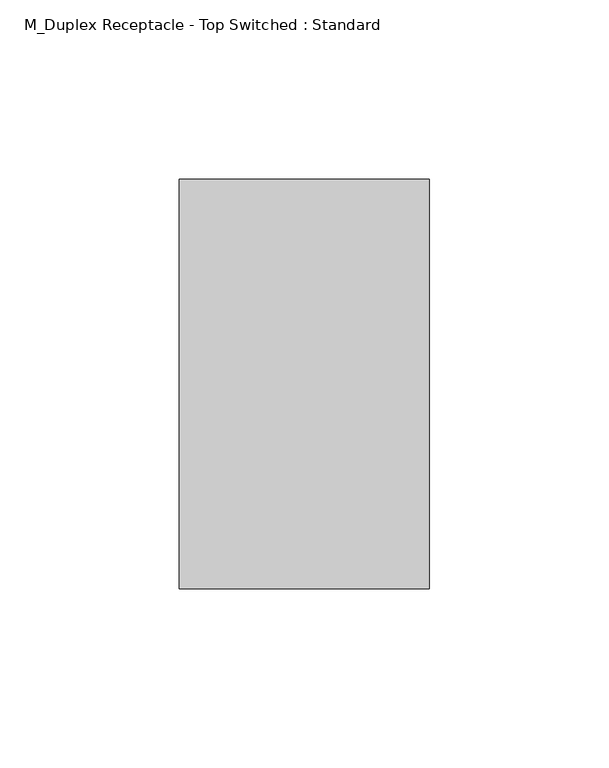
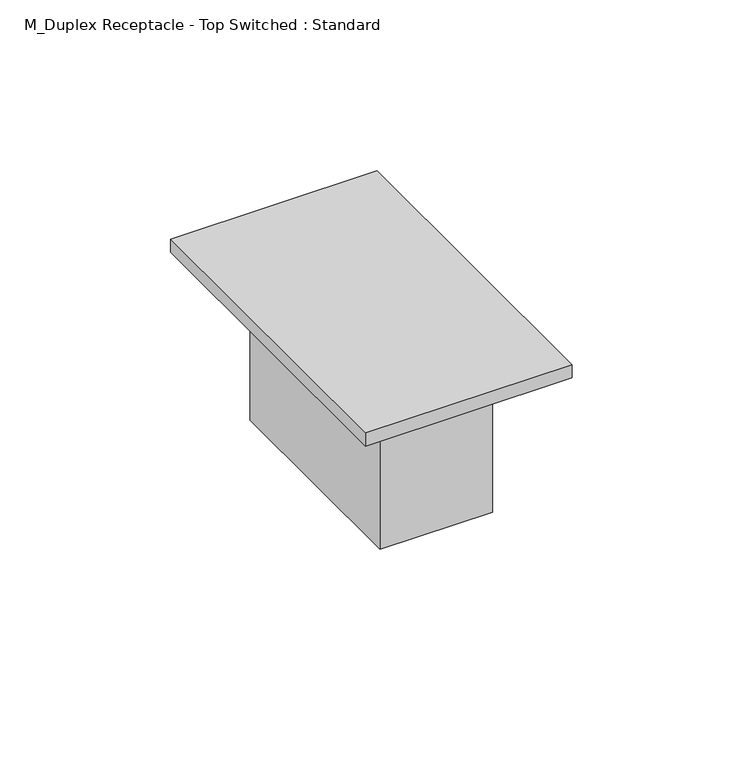
"""IFC4 building model written with IfcOpenShell, lengths in millimetres: proxy geometry, M_Duplex Receptacle - Top Switched : Standard."""

import ifcopenshell
import ifcopenshell.guid

model = None  # the IFC model being written
_history = None  # IfcOwnerHistory: only IFC2X3 demands one
_inside = {}  # id of a spatial element -> (the spatial element, [elements in it])
_under = {}  # id of a project, library or spatial element -> (it, [spatial elements below it])
_declared = {}  # id of a project -> (the project, [libraries it declares])
_typed = {}  # id of a type object -> (the type object, [elements of that type])
_made_of = {}  # id of a material, layer set ... -> (it, [elements and type objects made of it])


def new_model(schema):
    """Start an empty IFC model of exactly this schema.

    Asked for "IFC4X3", IfcOpenShell would pick the latest addendum, in which some entities
    have other attributes; the version numbers below select the first issue.
    IFC2X3 requires an IfcOwnerHistory on every rooted entity: one is made here for all.
    """
    global model, _history
    if schema == "IFC4X3":
        model = ifcopenshell.file(schema_version=(4, 3, 0, 0))
    else:
        model = ifcopenshell.file(schema=schema)
    _inside.clear()
    _under.clear()
    _declared.clear()
    _typed.clear()
    _made_of.clear()
    _history = None
    if model.schema == "IFC2X3":
        org = make("IfcOrganization", Name="unknown")
        user = make(
            "IfcPersonAndOrganization",
            ThePerson=make("IfcPerson", FamilyName="unknown"),
            TheOrganization=org,
        )
        app = make(
            "IfcApplication",
            ApplicationDeveloper=org,
            Version="unknown",
            ApplicationFullName="unknown",
            ApplicationIdentifier="unknown",
        )
        _history = make(
            "IfcOwnerHistory",
            OwningUser=user,
            OwningApplication=app,
            ChangeAction="ADDED",
            CreationDate=0,
        )
    return model


def make(cls, **values):
    """One entity of the class cls with the attributes given. An attribute that is None is left unset."""
    return model.create_entity(
        cls, **{name: value for name, value in values.items() if value is not None}
    )


def rooted(cls, **values):
    """An entity with a GlobalId (a new one), such as an element, a storey or a relation."""
    return make(cls, GlobalId=ifcopenshell.guid.new(), OwnerHistory=_history, **values)


def si_unit(unit_type, name, prefix=None):
    """IfcSIUnit, for example si_unit("LENGTHUNIT", "METRE", prefix="MILLI")."""
    return make("IfcSIUnit", UnitType=unit_type, Prefix=prefix, Name=name)


def assignment(units):
    """IfcUnitAssignment: the units of a project."""
    return None if units is None else make("IfcUnitAssignment", Units=units)


def point(xyz):
    """IfcCartesianPoint."""
    return None if xyz is None else make("IfcCartesianPoint", Coordinates=xyz)


def direction(xyz):
    """IfcDirection."""
    return None if xyz is None else make("IfcDirection", DirectionRatios=xyz)


def frame(location, z_axis=None, x_axis=None):
    """IfcAxis2Placement3D, a coordinate frame: its origin and axes. An axis left out is left unset."""
    return make(
        "IfcAxis2Placement3D",
        Location=point(location),
        Axis=direction(z_axis),
        RefDirection=direction(x_axis),
    )


def origin():
    """The frame at (0, 0, 0) with its axes left unset."""
    return frame((0.0, 0.0, 0.0))


def origin_with_axes():
    """The frame at (0, 0, 0) with the z axis (0, 0, 1) and the x axis (1, 0, 0) written out."""
    return frame((0.0, 0.0, 0.0), z_axis=(0.0, 0.0, 1.0), x_axis=(1.0, 0.0, 0.0))


def place(relative_to, where):
    """IfcLocalPlacement: puts the frame where relative to a parent placement (None: the world)."""
    return make(
        "IfcLocalPlacement", PlacementRelTo=relative_to, RelativePlacement=where
    )


def context(
    kind, dimensions, precision=None, world=None, true_north=None, identifier=None
):
    """IfcGeometricRepresentationContext, for example the 3D "Model" context."""
    return make(
        "IfcGeometricRepresentationContext",
        ContextIdentifier=identifier,
        ContextType=kind,
        CoordinateSpaceDimension=dimensions,
        Precision=precision,
        WorldCoordinateSystem=world,
        TrueNorth=true_north,
    )


def project(units=None, contexts=None):
    """IfcProject with its units and contexts."""
    return rooted(
        "IfcProject",
        Name="project",
        RepresentationContexts=contexts,
        UnitsInContext=assignment(units),
    )


def spatial(cls, under=None, at=None, **own):
    """A site, building, storey or space (cls), placed at a placement, below another one or the project."""
    s = rooted(cls, ObjectPlacement=at, **own)
    if under is not None:
        _under.setdefault(under.id(), (under, []))[1].append(s)
    return s


def polyline(points):
    """IfcPolyline through the points."""
    return make("IfcPolyline", Points=[point(p) for p in points])


def outline(outer, holes=None, kind="AREA"):
    """IfcArbitraryClosedProfileDef: a profile drawn as a closed curve; with holes, ...WithVoids."""
    if holes is None:
        return make("IfcArbitraryClosedProfileDef", ProfileType=kind, OuterCurve=outer)
    return make(
        "IfcArbitraryProfileDefWithVoids",
        ProfileType=kind,
        OuterCurve=outer,
        InnerCurves=holes,
    )


def extrude(swept, where, along, depth):
    """IfcExtrudedAreaSolid: the profile swept, set in the frame where, extruded along a direction by depth."""
    return make(
        "IfcExtrudedAreaSolid",
        SweptArea=swept,
        Position=where,
        ExtrudedDirection=direction(along),
        Depth=depth,
    )


def shape(context_of_items, identifier, shape_type, items):
    """IfcShapeRepresentation: the items that make up one representation, for example the "Body"."""
    return make(
        "IfcShapeRepresentation",
        ContextOfItems=context_of_items,
        RepresentationIdentifier=identifier,
        RepresentationType=shape_type,
        Items=items,
    )


def source(mapping_origin, context_of_items, identifier, shape_type, items):
    """IfcRepresentationMap: a shape defined once, which mapped items show again and again."""
    return make(
        "IfcRepresentationMap",
        MappingOrigin=mapping_origin,
        MappedRepresentation=shape(context_of_items, identifier, shape_type, items),
    )


def transform(
    local_origin,
    x_axis=None,
    y_axis=None,
    z_axis=None,
    scale=None,
    scale2=None,
    scale3=None,
    uniform=True,
):
    """IfcCartesianTransformationOperator3D, or its non-uniform kind. x_axis, y_axis, z_axis: its Axis1, 2, 3."""
    if uniform:
        return make(
            "IfcCartesianTransformationOperator3D",
            Axis1=direction(x_axis),
            Axis2=direction(y_axis),
            LocalOrigin=point(local_origin),
            Scale=scale,
            Axis3=direction(z_axis),
        )
    return make(
        "IfcCartesianTransformationOperator3DnonUniform",
        Axis1=direction(x_axis),
        Axis2=direction(y_axis),
        LocalOrigin=point(local_origin),
        Scale=scale,
        Axis3=direction(z_axis),
        Scale2=scale2,
        Scale3=scale3,
    )


def mapped(mapping_source, mapping_target):
    """IfcMappedItem: shows the shape of a source again, moved by a transform."""
    return make(
        "IfcMappedItem", MappingSource=mapping_source, MappingTarget=mapping_target
    )


def made_of(thing, what):
    """Note that an element or type object is made of a material, layer set ...; save() writes the relation."""
    if what is not None:
        _made_of.setdefault(what.id(), (what, []))[1].append(thing)
    return thing


def element(
    cls,
    number,
    at=None,
    inside=None,
    cuts=None,
    type_object=None,
    material=None,
    context=None,
    identifier="Body",
    shape_type=None,
    held_by="IfcProductDefinitionShape",
    body=None,
    shapes=None,
    **own,
):
    """One element of the class cls, such as IfcWall. Its Tag is "e" and its number.

    at: its placement. inside: the storey or other place that contains it. cuts: it is an
    opening in that element (IfcRelVoidsElement). A single representation is given by context,
    identifier, shape_type and body (its items); several are given by shapes. held_by: the class
    of the entity that holds the representations. save() writes the other relations.
    """
    e = rooted(cls, Tag="e%d" % number, ObjectPlacement=at, **own)
    if body is not None:
        shapes = [shape(context, identifier, shape_type, body)]
    if shapes is not None:
        e.Representation = make(held_by, Representations=shapes)
    if inside is not None:
        _inside.setdefault(inside.id(), (inside, []))[1].append(e)
    if cuts is not None:
        rooted(
            "IfcRelVoidsElement", RelatingBuildingElement=cuts, RelatedOpeningElement=e
        )
    if type_object is not None:
        _typed.setdefault(type_object.id(), (type_object, []))[1].append(e)
    return made_of(e, material)


def aggregate(whole, parts):
    """IfcRelAggregates: a whole, such as a stair, and the parts it consists of."""
    return rooted("IfcRelAggregates", RelatingObject=whole, RelatedObjects=parts)


def save(model, path):
    """Write the relations noted so far, then the file.

    IfcRelAggregates (storeys below a building ...), IfcRelContainedInSpatialStructure (elements
    in a storey), IfcRelDefinesByType, IfcRelAssociatesMaterial and IfcRelDeclares: one each for
    every whole, place, type object, material and project.
    """
    for whole, parts in _under.values():
        aggregate(whole, parts)
    for where, things in _inside.values():
        rooted(
            "IfcRelContainedInSpatialStructure",
            RelatedElements=things,
            RelatingStructure=where,
        )
    for kind, things in _typed.values():
        rooted("IfcRelDefinesByType", RelatedObjects=things, RelatingType=kind)
    for what, things in _made_of.values():
        rooted("IfcRelAssociatesMaterial", RelatedObjects=things, RelatingMaterial=what)
    for by, libraries in _declared.values():
        rooted("IfcRelDeclares", RelatingContext=by, RelatedDefinitions=libraries)
    model.write(path)


def m_duplex_receptacle_top_switched_standard_10251bba(model_context):
    return source(origin(), model_context, "Body", "SweptSolid", [
        extrude(outline(polyline([(19.05, 38.1), (19.05, -38.1), (-19.05, -38.1), (-19.05, 38.1), (19.05, 38.1)])), frame((0.0, 0.0, -53.975), z_axis=(0.0, 0.0, 1.0), x_axis=(1.0, 0.0, 0.0)), (0.0, 0.0, 1.0), 53.975),
        extrude(outline(polyline([(34.925, 57.15), (34.925, -57.15), (-34.925, -57.15), (-34.925, 57.15), (34.925, 57.15)])), origin_with_axes(), (0.0, 0.0, 1.0), 4.7625),
    ])


if __name__ == "__main__":
    model = new_model("IFC4")
    model_context = context("Model", 3, world=origin())
    ifc_project = project(units=[si_unit("LENGTHUNIT", "METRE", prefix="MILLI")], contexts=[model_context])
    site = spatial("IfcSite", under=ifc_project)
    building = spatial("IfcBuilding", under=site)
    placement = place(None, origin())
    m_duplex_receptacle_top_switched_standard_shape = m_duplex_receptacle_top_switched_standard_10251bba(model_context)
    element("IfcBuildingElementProxy", 1, Name="M_Duplex Receptacle - Top Switched : Standard", ObjectType="M_Duplex Receptacle - Top Switched : Standard", at=placement, inside=building, context=model_context, shape_type="MappedRepresentation", body=[
        mapped(m_duplex_receptacle_top_switched_standard_shape, transform((0.0, 0.0, 0.0), x_axis=(1.0, 0.0, 0.0), y_axis=(0.0, 1.0, 0.0), z_axis=(0.0, 0.0, 1.0))),
    ])
    save(model, "model.ifc")

# Revit data of these elements
# Type "M_Duplex Receptacle - Top Switched : Standard"
#   Type Mark = "M_Duplex Receptacle - Top Switched"
#   Classification.OmniClass.21.Number = "21-04 50 30 50"
#   Classification.MasterFormat.Description = "Wiring Devices"
#   Classification.OmniClass.22.Number = "22-26 27 26"
#   Classification.OmniClass.21.Description = "Wiring Devices"
#   Classification.UniFormat.II.Description = "Wiring Devices"
#   Classification.MasterFormat.Number = "26 27 26"
#   Classification.OmniClass.23.Number = "23-35 27 11"
#   Classification.OmniClass.22.Description = "Wiring Devices"
#   Classification.OmniClass.23.Description = "Electrical Receptacles"
#   Classification.UniFormat.II.Number = "D5030.50"
#   COBie.Type.CreatedBy = "info@mma.ie"
#   COBie.Type.CreatedOn = "2017-07-25T10:15:16"
#   COBie.Type.Name = "M_Duplex Receptacle - Top Switched"
#   COBie.Type.Category = "23-35 27 11 : Electrical Receptacles"
#   COBie.Type.Description = "M_Duplex Receptacle - Top Switched_Standard"
#   COBie.Type.AssetType = "Fixed"
#   COBie.Type.Manufacturer = ""
#   COBie.Type.ModelNumber = ""
#   Keynote = "26 27 26.B"
#   COBie.Type.ReplacementCost = 0
#   Switch Voltage = 220 V
#   Recep.Width = 69.85 mm
#   Recep.Load = 180 VA
#   Recep.Height = 114.3 mm
#   Load = 180 VA
#   Default Elevation = 460 mm
#   COBie.Type = yes
#   Recep.Material = Stainless Steel
#   Load Classification = Receptacle
#   Assembly Code = ""
# Materials
#   "Stainless Steel": class "Metal", colour RGB 120 120 120, transparency 0, Description = "Stainless Steel 18/8", Cost = 0
